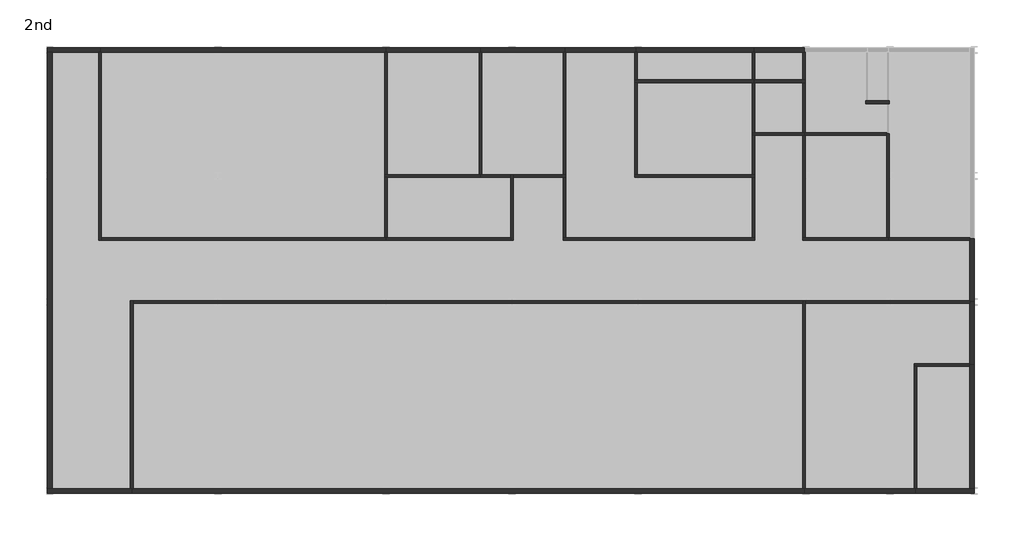
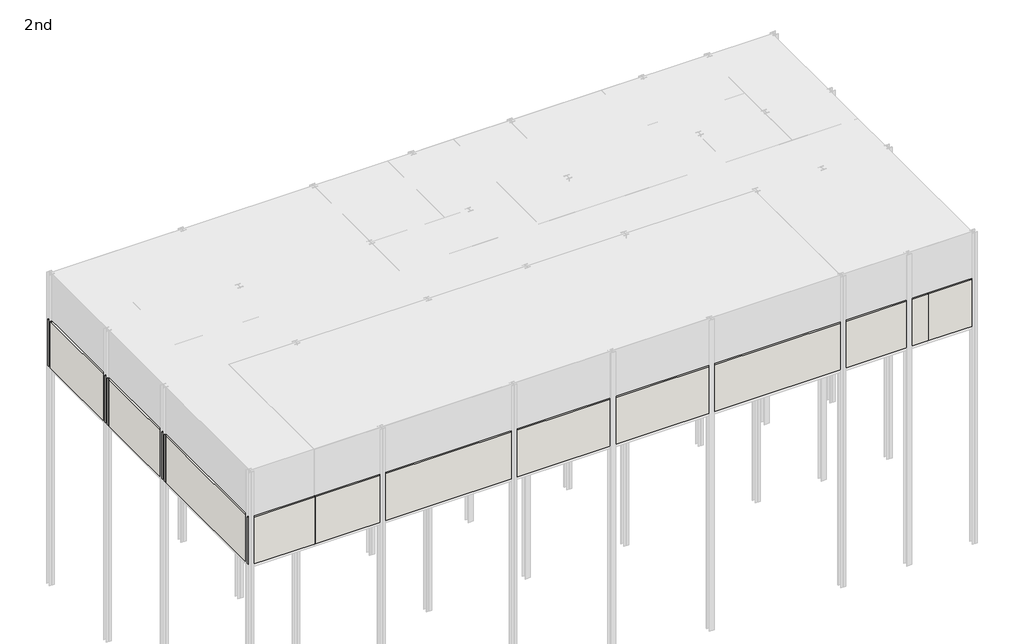
# One storey, part 1 of 3: 52 walls.
"""IFC4 building model written with IfcOpenShell, lengths in millimetres."""

from ifc_helpers import new_model, si_unit, frame, origin, place, context, project, spatial, polyline, outline, extrude, faceted_brep, element, save

model = new_model("IFC4")

# Units and contexts
model_context = context("Model", 3, world=origin())
ifc_project = project(units=[si_unit("LENGTHUNIT", "METRE", prefix="MILLI")], contexts=[model_context])

# Site, building, storey
site = spatial("IfcSite", under=ifc_project)
building = spatial("IfcBuilding", under=site)
storey = spatial("IfcBuildingStorey", under=building, Name="2nd", Elevation=14000.0)

# Walls
placement = place(None, origin())
element("IfcWall", 1, ObjectType="Wall-Ext_215Bwk", at=placement, inside=storey, context=model_context, shape_type="Brep", body=[
    faceted_brep([(160014.1020501, 130908.2581198, 14000.0), (192014.1020501, 130908.2581198, 14000.0), (192014.1020501, 130908.2581198, 17000.0), (160014.1020501, 130908.2581198, 17000.0), (160014.1020501, 131123.2581198, 14000.0), (160014.1020501, 131123.2581198, 17000.0), (160076.6020501, 131123.2581198, 17000.0), (191951.6020501, 131123.2581198, 17000.0), (192014.1020501, 131123.2581198, 17000.0), (192014.1020501, 131123.2581198, 14000.0), (191951.6020501, 131123.2581198, 14000.0), (160076.6020501, 131123.2581198, 14000.0)], [[[0, 1, 2, 3]], [[4, 5, 6, 7, 8, 9, 10, 11]], [[1, 0, 4, 11, 10, 9]], [[2, 1, 9, 8]], [[3, 2, 8, 7, 6, 5]], [[0, 3, 5, 4]]]),
])
element("IfcWall", 2, ObjectType="Wall-Ext_215Bwk", at=placement, inside=storey, context=model_context, shape_type="Brep", body=[
    faceted_brep([(172114.1020501, 152123.2581198, 14000.0), (158514.1020501, 152123.2581198, 14000.0), (158514.1020501, 152123.2581198, 17000.0), (172114.1020501, 152123.2581198, 17000.0), (172114.1020501, 151908.2581198, 14000.0), (172114.1020501, 151908.2581198, 17000.0), (172051.6020501, 151908.2581198, 17000.0), (158576.6020501, 151908.2581198, 17000.0), (158514.1020501, 151908.2581198, 17000.0), (158514.1020501, 151908.2581198, 14000.0), (158576.6020501, 151908.2581198, 14000.0), (172051.6020501, 151908.2581198, 14000.0)], [[[0, 1, 2, 3]], [[4, 5, 6, 7, 8, 9, 10, 11]], [[1, 0, 4, 11, 10, 9]], [[2, 1, 9, 8]], [[3, 2, 8, 7, 6, 5]], [[0, 3, 5, 4]]]),
])
element("IfcWall", 3, ObjectType="Wall-Ext_215Bwk", at=placement, inside=storey, context=model_context, shape_type="Brep", body=[
    faceted_brep([(176614.1020501, 152123.2581198, 14000.0), (172114.1020501, 152123.2581198, 14000.0), (172114.1020501, 152123.2581198, 17000.0), (176614.1020501, 152123.2581198, 17000.0), (176614.1020501, 151908.2581198, 14000.0), (176614.1020501, 151908.2581198, 17000.0), (176551.6020501, 151908.2581198, 17000.0), (172176.6020501, 151908.2581198, 17000.0), (172114.1020501, 151908.2581198, 17000.0), (172114.1020501, 151908.2581198, 14000.0), (172176.6020501, 151908.2581198, 14000.0), (176551.6020501, 151908.2581198, 14000.0)], [[[0, 1, 2, 3]], [[4, 5, 6, 7, 8, 9, 10, 11]], [[1, 0, 4, 11, 10, 9]], [[2, 1, 9, 8]], [[3, 2, 8, 7, 6, 5]], [[0, 3, 5, 4]]]),
])
element("IfcWall", 4, ObjectType="Wall-Ext_215Bwk", at=placement, inside=storey, context=model_context, shape_type="Brep", body=[
    faceted_brep([(180614.1020501, 152123.2581198, 14000.0), (176614.1020501, 152123.2581198, 14000.0), (176614.1020501, 152123.2581198, 17000.0), (180614.1020501, 152123.2581198, 17000.0), (180614.1020501, 151908.2581198, 14000.0), (180614.1020501, 151908.2581198, 17000.0), (180551.6020501, 151908.2581198, 17000.0), (176676.6020501, 151908.2581198, 17000.0), (176614.1020501, 151908.2581198, 17000.0), (176614.1020501, 151908.2581198, 14000.0), (176676.6020501, 151908.2581198, 14000.0), (180551.6020501, 151908.2581198, 14000.0)], [[[0, 1, 2, 3]], [[4, 5, 6, 7, 8, 9, 10, 11]], [[1, 0, 4, 11, 10, 9]], [[2, 1, 9, 8]], [[3, 2, 8, 7, 6, 5]], [[0, 3, 5, 4]]]),
])
element("IfcWall", 5, ObjectType="Wall-Ext_215Bwk", at=placement, inside=storey, context=model_context, shape_type="Brep", body=[
    faceted_brep([(192014.1020501, 152123.2581198, 14000.0), (189614.1020501, 152123.2581198, 14000.0), (189614.1020501, 152123.2581198, 17000.0), (192014.1020501, 152123.2581198, 17000.0), (192014.1020501, 151908.2581198, 14000.0), (192014.1020501, 151908.2581198, 17000.0), (191951.6020501, 151908.2581198, 17000.0), (189676.6020501, 151908.2581198, 17000.0), (189614.1020501, 151908.2581198, 17000.0), (189614.1020501, 151908.2581198, 14000.0), (189676.6020501, 151908.2581198, 14000.0), (191951.6020501, 151908.2581198, 14000.0)], [[[0, 1, 2, 3]], [[4, 5, 6, 7, 8, 9, 10, 11]], [[1, 0, 4, 11, 10, 9]], [[2, 1, 9, 8]], [[3, 2, 8, 7, 6, 5]], [[0, 3, 5, 4]]]),
])
element("IfcWall", 6, ObjectType="Wall-Ext_215Bwk", at=placement, inside=storey, context=model_context, shape_type="Brep", body=[
    faceted_brep([(200121.6020501, 140015.7581198, 14000.0), (200121.6020501, 143015.7581198, 14000.0), (200121.6020501, 143015.7581198, 17000.0), (200121.6020501, 140015.7581198, 17000.0), (199906.6020501, 140015.7581198, 14000.0), (199906.6020501, 140015.7581198, 17000.0), (199906.6020501, 140078.2581198, 17000.0), (199906.6020501, 142953.2581198, 17000.0), (199906.6020501, 143015.7581198, 17000.0), (199906.6020501, 143015.7581198, 14000.0), (199906.6020501, 142953.2581198, 14000.0), (199906.6020501, 140078.2581198, 14000.0)], [[[0, 1, 2, 3]], [[4, 5, 6, 7, 8, 9, 10, 11]], [[1, 0, 4, 11, 10, 9]], [[2, 1, 9, 8]], [[3, 2, 8, 7, 6, 5]], [[0, 3, 5, 4]]]),
])
element("IfcWall", 7, ObjectType="Wall-Ext_215Bwk", at=placement, inside=storey, context=model_context, shape_type="Brep", body=[
    faceted_brep([(158514.1020501, 152123.2581198, 14000.0), (156006.6020501, 152123.2581198, 14000.0), (156006.6020501, 152123.2581198, 17000.0), (158514.1020501, 152123.2581198, 17000.0), (158514.1020501, 151908.2581198, 14000.0), (158514.1020501, 151908.2581198, 17000.0), (158451.6020501, 151908.2581198, 17000.0), (156221.6020501, 151908.2581198, 17000.0), (156006.6020501, 151908.2581198, 17000.0), (156006.6020501, 151908.2581198, 14000.0), (156221.6020501, 151908.2581198, 14000.0), (158451.6020501, 151908.2581198, 14000.0)], [[[0, 1, 2, 3]], [[4, 5, 6, 7, 8, 9, 10, 11]], [[1, 0, 4, 11, 10, 9]], [[3, 2, 8, 7, 6, 5]], [[0, 3, 5, 4]], [[2, 1, 9, 8]]]),
])
element("IfcWall", 8, ObjectType="Wall-Ext_215Bwk", at=placement, inside=storey, context=model_context, shape_type="SweptSolid", body=[
    extrude(outline(polyline([(156006.6020501, 131123.2581198), (156006.6020501, 151908.2581198), (156221.6020501, 151908.2581198), (156221.6020501, 131123.2581198), (156006.6020501, 131123.2581198)])), frame((0.0, 0.0, 14000.0), z_axis=(0.0, 0.0, 1.0), x_axis=(1.0, 0.0, 0.0)), (0.0, 0.0, 1.0), 3000.0),
])
element("IfcWall", 9, ObjectType="Wall-Ext_215Bwk", at=placement, inside=storey, context=model_context, shape_type="Brep", body=[
    faceted_brep([(156006.6020501, 130908.2581198, 14000.0), (160014.1020501, 130908.2581198, 14000.0), (160014.1020501, 130908.2581198, 17000.0), (156006.6020501, 130908.2581198, 17000.0), (156006.6020501, 131123.2581198, 14000.0), (156006.6020501, 131123.2581198, 17000.0), (156221.6020501, 131123.2581198, 17000.0), (159951.6020501, 131123.2581198, 17000.0), (160014.1020501, 131123.2581198, 17000.0), (160014.1020501, 131123.2581198, 14000.0), (159951.6020501, 131123.2581198, 14000.0), (156221.6020501, 131123.2581198, 14000.0)], [[[0, 1, 2, 3]], [[4, 5, 6, 7, 8, 9, 10, 11]], [[1, 0, 4, 11, 10, 9]], [[2, 1, 9, 8]], [[3, 2, 8, 7, 6, 5]], [[0, 3, 5, 4]]]),
])
element("IfcWall", 10, ObjectType="Wall-Ext_215Bwk", at=placement, inside=storey, context=model_context, shape_type="Brep", body=[
    faceted_brep([(189614.1020501, 152123.2581198, 14000.0), (184014.1020501, 152123.2581198, 14000.0), (184014.1020501, 152123.2581198, 17000.0), (189614.1020501, 152123.2581198, 17000.0), (189614.1020501, 151908.2581198, 14000.0), (189614.1020501, 151908.2581198, 17000.0), (189551.6020501, 151908.2581198, 17000.0), (184076.6020501, 151908.2581198, 17000.0), (184014.1020501, 151908.2581198, 17000.0), (184014.1020501, 151908.2581198, 14000.0), (184076.6020501, 151908.2581198, 14000.0), (189551.6020501, 151908.2581198, 14000.0)], [[[0, 1, 2, 3]], [[4, 5, 6, 7, 8, 9, 10, 11]], [[1, 0, 4, 11, 10, 9]], [[2, 1, 9, 8]], [[3, 2, 8, 7, 6, 5]], [[0, 3, 5, 4]]]),
])
element("IfcWall", 11, ObjectType="Wall-Ext_215Bwk", at=placement, inside=storey, context=model_context, shape_type="Brep", body=[
    faceted_brep([(184014.1020501, 152123.2581198, 14000.0), (180614.1020501, 152123.2581198, 14000.0), (180614.1020501, 152123.2581198, 17000.0), (184014.1020501, 152123.2581198, 17000.0), (184014.1020501, 151908.2581198, 14000.0), (184014.1020501, 151908.2581198, 17000.0), (183951.6020501, 151908.2581198, 17000.0), (180676.6020501, 151908.2581198, 17000.0), (180614.1020501, 151908.2581198, 17000.0), (180614.1020501, 151908.2581198, 14000.0), (180676.6020501, 151908.2581198, 14000.0), (183951.6020501, 151908.2581198, 14000.0)], [[[0, 1, 2, 3]], [[4, 5, 6, 7, 8, 9, 10, 11]], [[1, 0, 4, 11, 10, 9]], [[2, 1, 9, 8]], [[3, 2, 8, 7, 6, 5]], [[0, 3, 5, 4]]]),
])
element("IfcWall", 12, ObjectType="Wall-Ext_215Bwk", at=placement, inside=storey, context=model_context, shape_type="Brep", body=[
    faceted_brep([(192014.1020501, 130908.2581198, 14000.0), (197314.1020501, 130908.2581198, 14000.0), (197314.1020501, 130908.2581198, 17000.0), (192014.1020501, 130908.2581198, 17000.0), (192014.1020501, 131123.2581198, 14000.0), (192014.1020501, 131123.2581198, 17000.0), (192076.6020501, 131123.2581198, 17000.0), (197251.6020501, 131123.2581198, 17000.0), (197314.1020501, 131123.2581198, 17000.0), (197314.1020501, 131123.2581198, 14000.0), (197251.6020501, 131123.2581198, 14000.0), (192076.6020501, 131123.2581198, 14000.0)], [[[0, 1, 2, 3]], [[4, 5, 6, 7, 8, 9, 10, 11]], [[1, 0, 4, 11, 10, 9]], [[2, 1, 9, 8]], [[3, 2, 8, 7, 6, 5]], [[0, 3, 5, 4]]]),
])
element("IfcWall", 13, ObjectType="Wall-Ext_215Bwk", at=placement, inside=storey, context=model_context, shape_type="Brep", body=[
    faceted_brep([(200121.6020501, 137015.7581198, 14000.0), (200121.6020501, 140015.7581198, 14000.0), (200121.6020501, 140015.7581198, 17000.0), (200121.6020501, 137015.7581198, 17000.0), (199906.6020501, 137015.7581198, 14000.0), (199906.6020501, 137015.7581198, 17000.0), (199906.6020501, 137078.2581198, 17000.0), (199906.6020501, 139953.2581198, 17000.0), (199906.6020501, 140015.7581198, 17000.0), (199906.6020501, 140015.7581198, 14000.0), (199906.6020501, 139953.2581198, 14000.0), (199906.6020501, 137078.2581198, 14000.0)], [[[0, 1, 2, 3]], [[4, 5, 6, 7, 8, 9, 10, 11]], [[1, 0, 4, 11, 10, 9]], [[2, 1, 9, 8]], [[3, 2, 8, 7, 6, 5]], [[0, 3, 5, 4]]]),
])
element("IfcWall", 14, ObjectType="Wall-Ext_215Bwk", at=placement, inside=storey, context=model_context, shape_type="Brep", body=[
    faceted_brep([(200121.6020501, 131123.2581198, 14000.0), (200121.6020501, 137015.7581198, 14000.0), (200121.6020501, 137015.7581198, 17000.0), (200121.6020501, 131123.2581198, 17000.0), (199906.6020501, 131123.2581198, 14000.0), (199906.6020501, 131123.2581198, 17000.0), (199906.6020501, 136953.2581198, 17000.0), (199906.6020501, 137015.7581198, 17000.0), (199906.6020501, 137015.7581198, 14000.0), (199906.6020501, 136953.2581198, 14000.0)], [[[0, 1, 2, 3]], [[4, 5, 6, 7, 8, 9]], [[1, 0, 4, 9, 8]], [[2, 1, 8, 7]], [[3, 2, 7, 6, 5]], [[0, 3, 5, 4]]]),
])
element("IfcWall", 15, ObjectType="Wall-Ext_215Bwk", at=placement, inside=storey, context=model_context, shape_type="Brep", body=[
    faceted_brep([(197314.1020501, 130908.2581198, 14000.0), (200121.6020501, 130908.2581198, 14000.0), (200121.6020501, 130908.2581198, 17000.0), (197314.1020501, 130908.2581198, 17000.0), (197314.1020501, 131123.2581198, 14000.0), (197314.1020501, 131123.2581198, 17000.0), (197376.6020501, 131123.2581198, 17000.0), (199906.6020501, 131123.2581198, 17000.0), (200121.6020501, 131123.2581198, 17000.0), (200121.6020501, 131123.2581198, 14000.0), (199906.6020501, 131123.2581198, 14000.0), (197376.6020501, 131123.2581198, 14000.0)], [[[0, 1, 2, 3]], [[4, 5, 6, 7, 8, 9, 10, 11]], [[1, 0, 4, 11, 10, 9]], [[3, 2, 8, 7, 6, 5]], [[0, 3, 5, 4]], [[2, 1, 9, 8]]]),
])
element("IfcWall", 16, ObjectType="Wall-Int_12P-100Blk-12P", at=placement, inside=storey, context=model_context, shape_type="SweptSolid", body=[
    extrude(outline(polyline([(160076.6020501, 140078.2581198), (191951.6020501, 140078.2581198), (191951.6020501, 139953.2581198), (160076.6020501, 139953.2581198), (160076.6020501, 140078.2581198)])), frame((0.0, 0.0, 14000.0), z_axis=(0.0, 0.0, 1.0), x_axis=(1.0, 0.0, 0.0)), (0.0, 0.0, 1.0), 3000.0),
])
element("IfcWall", 17, ObjectType="Wall-Int_12P-100Blk-12P", at=placement, inside=storey, context=model_context, shape_type="Brep", body=[
    faceted_brep([(159951.6020501, 140078.2581198, 14000.0), (159951.6020501, 131123.2581198, 14000.0), (159951.6020501, 131123.2581198, 17000.0), (159951.6020501, 140078.2581198, 17000.0), (160076.6020501, 140078.2581198, 14000.0), (160076.6020501, 140078.2581198, 17000.0), (160076.6020501, 139953.2581198, 17000.0), (160076.6020501, 131123.2581198, 17000.0), (160076.6020501, 131123.2581198, 14000.0), (160076.6020501, 139953.2581198, 14000.0), (160014.1020501, 131123.2581198, 14000.0), (160014.1020501, 131123.2581198, 17000.0)], [[[0, 1, 2, 3]], [[4, 5, 6, 7, 8, 9]], [[1, 0, 4, 9, 8, 10]], [[3, 2, 11, 7, 6, 5]], [[0, 3, 5, 4]], [[2, 1, 10, 8, 7, 11]]]),
])
element("IfcWall", 18, ObjectType="Wall-Int_12P-100Blk-12P", at=placement, inside=storey, context=model_context, shape_type="Brep", body=[
    faceted_brep([(192076.6020501, 131123.2581198, 14000.0), (192076.6020501, 139953.2581198, 14000.0), (192076.6020501, 140078.2581198, 14000.0), (192076.6020501, 140078.2581198, 17000.0), (192076.6020501, 139953.2581198, 17000.0), (192076.6020501, 131123.2581198, 17000.0), (191951.6020501, 131123.2581198, 14000.0), (191951.6020501, 131123.2581198, 17000.0), (191951.6020501, 139953.2581198, 17000.0), (191951.6020501, 140078.2581198, 17000.0), (191951.6020501, 140078.2581198, 14000.0), (191951.6020501, 139953.2581198, 14000.0), (192014.1020501, 131123.2581198, 14000.0), (192014.1020501, 131123.2581198, 17000.0)], [[[0, 1, 2, 3, 4, 5]], [[6, 7, 8, 9, 10, 11]], [[2, 1, 0, 12, 6, 11, 10]], [[5, 4, 3, 9, 8, 7, 13]], [[3, 2, 10, 9]], [[0, 5, 13, 7, 6, 12]]]),
])
element("IfcWall", 19, ObjectType="Wall-Int_12P-100Blk-12P", at=placement, inside=storey, context=model_context, shape_type="Brep", body=[
    faceted_brep([(158451.6020501, 151908.2581198, 14000.0), (158451.6020501, 142953.2581198, 14000.0), (158451.6020501, 142953.2581198, 17000.0), (158451.6020501, 151908.2581198, 17000.0), (158576.6020501, 151908.2581198, 14000.0), (158576.6020501, 151908.2581198, 17000.0), (158576.6020501, 143078.2581198, 17000.0), (158576.6020501, 142953.2581198, 17000.0), (158576.6020501, 142953.2581198, 14000.0), (158576.6020501, 143078.2581198, 14000.0), (158514.1020501, 151908.2581198, 14000.0), (158514.1020501, 151908.2581198, 17000.0)], [[[0, 1, 2, 3]], [[4, 5, 6, 7, 8, 9]], [[1, 0, 10, 4, 9, 8]], [[3, 2, 7, 6, 5, 11]], [[0, 3, 11, 5, 4, 10]], [[2, 1, 8, 7]]]),
])
element("IfcWall", 20, ObjectType="Wall-Int_12P-100Blk-12P", at=placement, inside=storey, context=model_context, shape_type="Brep", body=[
    faceted_brep([(158576.6020501, 142953.2581198, 14000.0), (172114.1020501, 142953.2581198, 14000.0), (172114.1020501, 142953.2581198, 17000.0), (158576.6020501, 142953.2581198, 17000.0), (158576.6020501, 143078.2581198, 14000.0), (158576.6020501, 143078.2581198, 17000.0), (172051.6020501, 143078.2581198, 17000.0), (172114.1020501, 143078.2581198, 17000.0), (172114.1020501, 143078.2581198, 14000.0), (172051.6020501, 143078.2581198, 14000.0)], [[[0, 1, 2, 3]], [[4, 5, 6, 7, 8, 9]], [[1, 0, 4, 9, 8]], [[2, 1, 8, 7]], [[3, 2, 7, 6, 5]], [[0, 3, 5, 4]]]),
])
element("IfcWall", 21, ObjectType="Wall-Int_12P-100Blk-12P", at=placement, inside=storey, context=model_context, shape_type="Brep", body=[
    faceted_brep([(172176.6020501, 143078.2581198, 14000.0), (172176.6020501, 145953.2581198, 14000.0), (172176.6020501, 145953.2581198, 17000.0), (172176.6020501, 143078.2581198, 17000.0), (172051.6020501, 143078.2581198, 14000.0), (172051.6020501, 143078.2581198, 17000.0), (172051.6020501, 145953.2581198, 17000.0), (172051.6020501, 145953.2581198, 14000.0), (172114.1020501, 143078.2581198, 14000.0), (172114.1020501, 143078.2581198, 17000.0)], [[[0, 1, 2, 3]], [[4, 5, 6, 7]], [[1, 0, 8, 4, 7]], [[3, 2, 6, 5, 9]], [[0, 3, 9, 5, 4, 8]], [[2, 1, 7, 6]]]),
])
element("IfcWall", 22, ObjectType="Wall-Int_12P-100Blk-12P", at=placement, inside=storey, context=model_context, shape_type="Brep", body=[
    faceted_brep([(172176.6020501, 146078.2581198, 14000.0), (172176.6020501, 151908.2581198, 14000.0), (172176.6020501, 151908.2581198, 17000.0), (172176.6020501, 146078.2581198, 17000.0), (172051.6020501, 146078.2581198, 14000.0), (172051.6020501, 146078.2581198, 17000.0), (172051.6020501, 151908.2581198, 17000.0), (172051.6020501, 151908.2581198, 14000.0), (172114.1020501, 151908.2581198, 14000.0), (172114.1020501, 151908.2581198, 17000.0)], [[[0, 1, 2, 3]], [[4, 5, 6, 7]], [[1, 0, 4, 7, 8]], [[3, 2, 9, 6, 5]], [[2, 1, 8, 7, 6, 9]], [[0, 3, 5, 4]]]),
])
element("IfcWall", 23, ObjectType="Wall-Int_12P-100Blk-12P", at=placement, inside=storey, context=model_context, shape_type="Brep", body=[
    faceted_brep([(172051.6020501, 145953.2581198, 14000.0), (172176.6020501, 145953.2581198, 14000.0), (176614.1020501, 145953.2581198, 14000.0), (176614.1020501, 145953.2581198, 17000.0), (172176.6020501, 145953.2581198, 17000.0), (172051.6020501, 145953.2581198, 17000.0), (172051.6020501, 146078.2581198, 14000.0), (172051.6020501, 146078.2581198, 17000.0), (172176.6020501, 146078.2581198, 17000.0), (176551.6020501, 146078.2581198, 17000.0), (176614.1020501, 146078.2581198, 17000.0), (176614.1020501, 146078.2581198, 14000.0), (176551.6020501, 146078.2581198, 14000.0), (172176.6020501, 146078.2581198, 14000.0)], [[[0, 1, 2, 3, 4, 5]], [[6, 7, 8, 9, 10, 11, 12, 13]], [[2, 1, 0, 6, 13, 12, 11]], [[3, 2, 11, 10]], [[5, 4, 3, 10, 9, 8, 7]], [[0, 5, 7, 6]]]),
])
element("IfcWall", 24, ObjectType="Wall-Int_12P-100Blk-12P", at=placement, inside=storey, context=model_context, shape_type="Brep", body=[
    faceted_brep([(176676.6020501, 146078.2581198, 14000.0), (176676.6020501, 151908.2581198, 14000.0), (176676.6020501, 151908.2581198, 17000.0), (176676.6020501, 146078.2581198, 17000.0), (176551.6020501, 146078.2581198, 14000.0), (176551.6020501, 146078.2581198, 17000.0), (176551.6020501, 151908.2581198, 17000.0), (176551.6020501, 151908.2581198, 14000.0), (176614.1020501, 146078.2581198, 14000.0), (176614.1020501, 151908.2581198, 14000.0), (176614.1020501, 151908.2581198, 17000.0), (176614.1020501, 146078.2581198, 17000.0)], [[[0, 1, 2, 3]], [[4, 5, 6, 7]], [[1, 0, 8, 4, 7, 9]], [[3, 2, 10, 6, 5, 11]], [[2, 1, 9, 7, 6, 10]], [[0, 3, 11, 5, 4, 8]]]),
])
element("IfcWall", 25, ObjectType="Wall-Int_12P-100Blk-12P", at=placement, inside=storey, context=model_context, shape_type="Brep", body=[
    faceted_brep([(191951.6020501, 147953.2581198, 14000.0), (191951.6020501, 143078.2581198, 14000.0), (191951.6020501, 143078.2581198, 17000.0), (191951.6020501, 147953.2581198, 17000.0), (192076.6020501, 147953.2581198, 14000.0), (192076.6020501, 147953.2581198, 17000.0), (192076.6020501, 143078.2581198, 17000.0), (192076.6020501, 143078.2581198, 14000.0), (192014.1020501, 147953.2581198, 14000.0), (192014.1020501, 147953.2581198, 17000.0)], [[[0, 1, 2, 3]], [[4, 5, 6, 7]], [[1, 0, 8, 4, 7]], [[3, 2, 6, 5, 9]], [[0, 3, 9, 5, 4, 8]], [[2, 1, 7, 6]]]),
])
element("IfcWall", 26, ObjectType="Wall-Int_12P-100Blk-12P", at=placement, inside=storey, context=model_context, shape_type="Brep", body=[
    faceted_brep([(191951.6020501, 142953.2581198, 14000.0), (196014.1020501, 142953.2581198, 14000.0), (196014.1020501, 142953.2581198, 17000.0), (191951.6020501, 142953.2581198, 17000.0), (191951.6020501, 143078.2581198, 14000.0), (191951.6020501, 143078.2581198, 17000.0), (192076.6020501, 143078.2581198, 17000.0), (195951.6020501, 143078.2581198, 17000.0), (196014.1020501, 143078.2581198, 17000.0), (196014.1020501, 143078.2581198, 14000.0), (195951.6020501, 143078.2581198, 14000.0), (192076.6020501, 143078.2581198, 14000.0)], [[[0, 1, 2, 3]], [[4, 5, 6, 7, 8, 9, 10, 11]], [[1, 0, 4, 11, 10, 9]], [[2, 1, 9, 8]], [[3, 2, 8, 7, 6, 5]], [[0, 3, 5, 4]]]),
])
element("IfcWall", 27, ObjectType="Wall-Int_12P-100Blk-12P", at=placement, inside=storey, context=model_context, shape_type="Brep", body=[
    faceted_brep([(196076.6020501, 143078.2581198, 14000.0), (196076.6020501, 148015.7581198, 14000.0), (196076.6020501, 148015.7581198, 17000.0), (196076.6020501, 143078.2581198, 17000.0), (195951.6020501, 143078.2581198, 14000.0), (195951.6020501, 143078.2581198, 17000.0), (195951.6020501, 147953.2581198, 17000.0), (195951.6020501, 148015.7581198, 17000.0), (195951.6020501, 148015.7581198, 14000.0), (195951.6020501, 147953.2581198, 14000.0), (196014.1020501, 143078.2581198, 14000.0), (196014.1020501, 143078.2581198, 17000.0)], [[[0, 1, 2, 3]], [[4, 5, 6, 7, 8, 9]], [[1, 0, 10, 4, 9, 8]], [[2, 1, 8, 7]], [[3, 2, 7, 6, 5, 11]], [[0, 3, 11, 5, 4, 10]]]),
])
element("IfcWall", 28, ObjectType="Wall-Int_12P-100Blk-12P", at=placement, inside=storey, context=model_context, shape_type="Brep", body=[
    faceted_brep([(195951.6020501, 148078.2581198, 14000.0), (192076.6020501, 148078.2581198, 14000.0), (192014.1020501, 148078.2581198, 14000.0), (192014.1020501, 148078.2581198, 17000.0), (192076.6020501, 148078.2581198, 17000.0), (195951.6020501, 148078.2581198, 17000.0), (195951.6020501, 147953.2581198, 14000.0), (195951.6020501, 147953.2581198, 17000.0), (192076.6020501, 147953.2581198, 17000.0), (192014.1020501, 147953.2581198, 17000.0), (192014.1020501, 147953.2581198, 14000.0), (192076.6020501, 147953.2581198, 14000.0), (195951.6020501, 148015.7581198, 14000.0), (195951.6020501, 148015.7581198, 17000.0)], [[[0, 1, 2, 3, 4, 5]], [[6, 7, 8, 9, 10, 11]], [[2, 1, 0, 12, 6, 11, 10]], [[3, 2, 10, 9]], [[5, 4, 3, 9, 8, 7, 13]], [[0, 5, 13, 7, 6, 12]]]),
])
element("IfcWall", 29, ObjectType="Wall-Int_12P-100Blk-12P", at=placement, inside=storey, context=model_context, shape_type="Brep", body=[
    faceted_brep([(196014.1020501, 142953.2581198, 14000.0), (199906.6020501, 142953.2581198, 14000.0), (199906.6020501, 142953.2581198, 17000.0), (196014.1020501, 142953.2581198, 17000.0), (196014.1020501, 143078.2581198, 14000.0), (196014.1020501, 143078.2581198, 17000.0), (196076.6020501, 143078.2581198, 17000.0), (199906.6020501, 143078.2581198, 17000.0), (199906.6020501, 143078.2581198, 14000.0), (196076.6020501, 143078.2581198, 14000.0), (199906.6020501, 143015.7581198, 14000.0), (199906.6020501, 143015.7581198, 17000.0)], [[[0, 1, 2, 3]], [[4, 5, 6, 7, 8, 9]], [[1, 0, 4, 9, 8, 10]], [[3, 2, 11, 7, 6, 5]], [[0, 3, 5, 4]], [[2, 1, 10, 8, 7, 11]]]),
])
element("IfcWall", 30, ObjectType="Wall-Int_12P-100Blk-12P", at=placement, inside=storey, context=model_context, shape_type="Brep", body=[
    faceted_brep([(176614.1020501, 145953.2581198, 14000.0), (178051.6020501, 145953.2581198, 14000.0), (178051.6020501, 145953.2581198, 17000.0), (176614.1020501, 145953.2581198, 17000.0), (176614.1020501, 146078.2581198, 14000.0), (176614.1020501, 146078.2581198, 17000.0), (176676.6020501, 146078.2581198, 17000.0), (178051.6020501, 146078.2581198, 17000.0), (178051.6020501, 146078.2581198, 14000.0), (176676.6020501, 146078.2581198, 14000.0)], [[[0, 1, 2, 3]], [[4, 5, 6, 7, 8, 9]], [[1, 0, 4, 9, 8]], [[3, 2, 7, 6, 5]], [[0, 3, 5, 4]], [[2, 1, 8, 7]]]),
])
element("IfcWall", 31, ObjectType="Wall-Int_12P-100Blk-12P", at=placement, inside=storey, context=model_context, shape_type="Brep", body=[
    faceted_brep([(178176.6020501, 145953.2581198, 14000.0), (180551.6020501, 145953.2581198, 14000.0), (180676.6020501, 145953.2581198, 14000.0), (180676.6020501, 145953.2581198, 17000.0), (180551.6020501, 145953.2581198, 17000.0), (178176.6020501, 145953.2581198, 17000.0), (178176.6020501, 146078.2581198, 14000.0), (178176.6020501, 146078.2581198, 17000.0), (180551.6020501, 146078.2581198, 17000.0), (180676.6020501, 146078.2581198, 17000.0), (180676.6020501, 146078.2581198, 14000.0), (180551.6020501, 146078.2581198, 14000.0)], [[[0, 1, 2, 3, 4, 5]], [[6, 7, 8, 9, 10, 11]], [[2, 1, 0, 6, 11, 10]], [[5, 4, 3, 9, 8, 7]], [[3, 2, 10, 9]], [[0, 5, 7, 6]]]),
])
element("IfcWall", 32, ObjectType="Wall-Int_12P-100Blk-12P", at=placement, inside=storey, context=model_context, shape_type="Brep", body=[
    faceted_brep([(180676.6020501, 146078.2581198, 14000.0), (180676.6020501, 151908.2581198, 14000.0), (180676.6020501, 151908.2581198, 17000.0), (180676.6020501, 146078.2581198, 17000.0), (180551.6020501, 146078.2581198, 14000.0), (180551.6020501, 146078.2581198, 17000.0), (180551.6020501, 151908.2581198, 17000.0), (180551.6020501, 151908.2581198, 14000.0), (180614.1020501, 151908.2581198, 14000.0), (180614.1020501, 151908.2581198, 17000.0)], [[[0, 1, 2, 3]], [[4, 5, 6, 7]], [[1, 0, 4, 7, 8]], [[3, 2, 9, 6, 5]], [[2, 1, 8, 7, 6, 9]], [[0, 3, 5, 4]]]),
])
element("IfcWall", 33, ObjectType="Wall-Int_12P-100Blk-12P", at=placement, inside=storey, context=model_context, shape_type="Brep", body=[
    faceted_brep([(172114.1020501, 142953.2581198, 14000.0), (178051.6020501, 142953.2581198, 14000.0), (178051.6020501, 142953.2581198, 17000.0), (172114.1020501, 142953.2581198, 17000.0), (172114.1020501, 143078.2581198, 14000.0), (172114.1020501, 143078.2581198, 17000.0), (172176.6020501, 143078.2581198, 17000.0), (178051.6020501, 143078.2581198, 17000.0), (178051.6020501, 143078.2581198, 14000.0), (172176.6020501, 143078.2581198, 14000.0)], [[[0, 1, 2, 3]], [[4, 5, 6, 7, 8, 9]], [[1, 0, 4, 9, 8]], [[3, 2, 7, 6, 5]], [[0, 3, 5, 4]], [[2, 1, 8, 7]]]),
])
element("IfcWall", 34, ObjectType="Wall-Int_12P-100Blk-12P", at=placement, inside=storey, context=model_context, shape_type="Brep", body=[
    faceted_brep([(178176.6020501, 142953.2581198, 14000.0), (178176.6020501, 145953.2581198, 14000.0), (178176.6020501, 146078.2581198, 14000.0), (178176.6020501, 146078.2581198, 17000.0), (178176.6020501, 145953.2581198, 17000.0), (178176.6020501, 142953.2581198, 17000.0), (178051.6020501, 142953.2581198, 14000.0), (178051.6020501, 142953.2581198, 17000.0), (178051.6020501, 143078.2581198, 17000.0), (178051.6020501, 145953.2581198, 17000.0), (178051.6020501, 146078.2581198, 17000.0), (178051.6020501, 146078.2581198, 14000.0), (178051.6020501, 145953.2581198, 14000.0), (178051.6020501, 143078.2581198, 14000.0)], [[[0, 1, 2, 3, 4, 5]], [[6, 7, 8, 9, 10, 11, 12, 13]], [[2, 1, 0, 6, 13, 12, 11]], [[5, 4, 3, 10, 9, 8, 7]], [[0, 5, 7, 6]], [[3, 2, 11, 10]]]),
])
element("IfcWall", 35, ObjectType="Wall-Int_12P-100Blk-12P", at=placement, inside=storey, context=model_context, shape_type="Brep", body=[
    faceted_brep([(189551.6020501, 151908.2581198, 14000.0), (189551.6020501, 150578.2581198, 14000.0), (189551.6020501, 150578.2581198, 17000.0), (189551.6020501, 151908.2581198, 17000.0), (189676.6020501, 151908.2581198, 14000.0), (189676.6020501, 151908.2581198, 17000.0), (189676.6020501, 150578.2581198, 17000.0), (189676.6020501, 150578.2581198, 14000.0), (189614.1020501, 151908.2581198, 14000.0), (189614.1020501, 150578.2581198, 14000.0), (189614.1020501, 150578.2581198, 17000.0), (189614.1020501, 151908.2581198, 17000.0)], [[[0, 1, 2, 3]], [[4, 5, 6, 7]], [[1, 0, 8, 4, 7, 9]], [[3, 2, 10, 6, 5, 11]], [[0, 3, 11, 5, 4, 8]], [[2, 1, 9, 7, 6, 10]]]),
])
element("IfcWall", 36, ObjectType="Wall-Int_12P-100Blk-12P", at=placement, inside=storey, context=model_context, shape_type="Brep", body=[
    faceted_brep([(189614.1020501, 150453.2581198, 14000.0), (189676.6020501, 150453.2581198, 14000.0), (191951.6020501, 150453.2581198, 14000.0), (192076.6020501, 150453.2581198, 14000.0), (192076.6020501, 150453.2581198, 17000.0), (191951.6020501, 150453.2581198, 17000.0), (189676.6020501, 150453.2581198, 17000.0), (189614.1020501, 150453.2581198, 17000.0), (189614.1020501, 150578.2581198, 14000.0), (189614.1020501, 150578.2581198, 17000.0), (189676.6020501, 150578.2581198, 17000.0), (191951.6020501, 150578.2581198, 17000.0), (192076.6020501, 150578.2581198, 17000.0), (192076.6020501, 150578.2581198, 14000.0), (191951.6020501, 150578.2581198, 14000.0), (189676.6020501, 150578.2581198, 14000.0)], [[[0, 1, 2, 3, 4, 5, 6, 7]], [[8, 9, 10, 11, 12, 13, 14, 15]], [[3, 2, 1, 0, 8, 15, 14, 13]], [[7, 6, 5, 4, 12, 11, 10, 9]], [[0, 7, 9, 8]], [[4, 3, 13, 12]]]),
])
element("IfcWall", 37, ObjectType="Wall-Int_12P-100Blk-12P", at=placement, inside=storey, context=model_context, shape_type="Brep", body=[
    faceted_brep([(192076.6020501, 150578.2581198, 14000.0), (192076.6020501, 151908.2581198, 14000.0), (192076.6020501, 151908.2581198, 17000.0), (192076.6020501, 150578.2581198, 17000.0), (191951.6020501, 150578.2581198, 14000.0), (191951.6020501, 150578.2581198, 17000.0), (191951.6020501, 151908.2581198, 17000.0), (191951.6020501, 151908.2581198, 14000.0), (192014.1020501, 151908.2581198, 14000.0), (192014.1020501, 151908.2581198, 17000.0)], [[[0, 1, 2, 3]], [[4, 5, 6, 7]], [[1, 0, 4, 7, 8]], [[3, 2, 9, 6, 5]], [[2, 1, 8, 7, 6, 9]], [[0, 3, 5, 4]]]),
])
element("IfcWall", 38, ObjectType="Wall-Int_12P-100Blk-12P", at=placement, inside=storey, context=model_context, shape_type="Brep", body=[
    faceted_brep([(192076.6020501, 139953.2581198, 14000.0), (199906.6020501, 139953.2581198, 14000.0), (199906.6020501, 139953.2581198, 17000.0), (192076.6020501, 139953.2581198, 17000.0), (192076.6020501, 140078.2581198, 14000.0), (192076.6020501, 140078.2581198, 17000.0), (199906.6020501, 140078.2581198, 17000.0), (199906.6020501, 140078.2581198, 14000.0), (199906.6020501, 140015.7581198, 14000.0), (199906.6020501, 140015.7581198, 17000.0)], [[[0, 1, 2, 3]], [[4, 5, 6, 7]], [[1, 0, 4, 7, 8]], [[3, 2, 9, 6, 5]], [[0, 3, 5, 4]], [[2, 1, 8, 7, 6, 9]]]),
])
element("IfcWall", 39, ObjectType="Wall-Int_12P-100Blk-12P", at=placement, inside=storey, context=model_context, shape_type="Brep", body=[
    faceted_brep([(192014.1020501, 148078.2581198, 14000.0), (191951.6020501, 148078.2581198, 14000.0), (189676.6020501, 148078.2581198, 14000.0), (189551.6020501, 148078.2581198, 14000.0), (189551.6020501, 148078.2581198, 17000.0), (189676.6020501, 148078.2581198, 17000.0), (191951.6020501, 148078.2581198, 17000.0), (192014.1020501, 148078.2581198, 17000.0), (192014.1020501, 147953.2581198, 14000.0), (192014.1020501, 147953.2581198, 17000.0), (191951.6020501, 147953.2581198, 17000.0), (189676.6020501, 147953.2581198, 17000.0), (189551.6020501, 147953.2581198, 17000.0), (189551.6020501, 147953.2581198, 14000.0), (189676.6020501, 147953.2581198, 14000.0), (191951.6020501, 147953.2581198, 14000.0)], [[[0, 1, 2, 3, 4, 5, 6, 7]], [[8, 9, 10, 11, 12, 13, 14, 15]], [[3, 2, 1, 0, 8, 15, 14, 13]], [[7, 6, 5, 4, 12, 11, 10, 9]], [[0, 7, 9, 8]], [[4, 3, 13, 12]]]),
])
element("IfcWall", 40, ObjectType="Wall-Int_12P-100Blk-12P", at=placement, inside=storey, context=model_context, shape_type="SweptSolid", body=[
    extrude(outline(polyline([(189551.6020501, 146078.2581198), (189551.6020501, 147953.2581198), (189676.6020501, 147953.2581198), (189676.6020501, 146078.2581198), (189551.6020501, 146078.2581198)])), frame((0.0, 0.0, 14000.0), z_axis=(0.0, 0.0, 1.0), x_axis=(1.0, 0.0, 0.0)), (0.0, 0.0, 1.0), 3000.0),
])
element("IfcWall", 41, ObjectType="Wall-Int_12P-100Blk-12P", at=placement, inside=storey, context=model_context, shape_type="SweptSolid", body=[
    extrude(outline(polyline([(189551.6020501, 143078.2581198), (189551.6020501, 145953.2581198), (189676.6020501, 145953.2581198), (189676.6020501, 143078.2581198), (189551.6020501, 143078.2581198)])), frame((0.0, 0.0, 14000.0), z_axis=(0.0, 0.0, 1.0), x_axis=(1.0, 0.0, 0.0)), (0.0, 0.0, 1.0), 3000.0),
])
element("IfcWall", 42, ObjectType="Wall-Int_12P-100Blk-12P", at=placement, inside=storey, context=model_context, shape_type="Brep", body=[
    faceted_brep([(189676.6020501, 143078.2581198, 14000.0), (189551.6020501, 143078.2581198, 14000.0), (180676.6020501, 143078.2581198, 14000.0), (180551.6020501, 143078.2581198, 14000.0), (180551.6020501, 143078.2581198, 17000.0), (180676.6020501, 143078.2581198, 17000.0), (189551.6020501, 143078.2581198, 17000.0), (189676.6020501, 143078.2581198, 17000.0), (189676.6020501, 142953.2581198, 14000.0), (189676.6020501, 142953.2581198, 17000.0), (180551.6020501, 142953.2581198, 17000.0), (180551.6020501, 142953.2581198, 14000.0)], [[[0, 1, 2, 3, 4, 5, 6, 7]], [[8, 9, 10, 11]], [[3, 2, 1, 0, 8, 11]], [[7, 6, 5, 4, 10, 9]], [[0, 7, 9, 8]], [[4, 3, 11, 10]]]),
])
element("IfcWall", 43, ObjectType="Wall-Int_12P-100Blk-12P", at=placement, inside=storey, context=model_context, shape_type="SweptSolid", body=[
    extrude(outline(polyline([(180676.6020501, 145953.2581198), (180676.6020501, 143078.2581198), (180551.6020501, 143078.2581198), (180551.6020501, 145953.2581198), (180676.6020501, 145953.2581198)])), frame((0.0, 0.0, 14000.0), z_axis=(0.0, 0.0, 1.0), x_axis=(1.0, 0.0, 0.0)), (0.0, 0.0, 1.0), 3000.0),
])
element("IfcWall", 44, ObjectType="Wall-Int_12P-100Blk-12P", at=placement, inside=storey, context=model_context, shape_type="Brep", body=[
    faceted_brep([(189551.6020501, 150453.2581198, 14000.0), (189551.6020501, 148078.2581198, 14000.0), (189551.6020501, 148078.2581198, 17000.0), (189551.6020501, 150453.2581198, 17000.0), (189676.6020501, 150453.2581198, 14000.0), (189676.6020501, 150453.2581198, 17000.0), (189676.6020501, 148078.2581198, 17000.0), (189676.6020501, 148078.2581198, 14000.0), (189614.1020501, 150453.2581198, 14000.0), (189614.1020501, 150453.2581198, 17000.0)], [[[0, 1, 2, 3]], [[4, 5, 6, 7]], [[1, 0, 8, 4, 7]], [[3, 2, 6, 5, 9]], [[0, 3, 9, 5, 4, 8]], [[2, 1, 7, 6]]]),
])
element("IfcWall", 45, ObjectType="Wall-Int_12P-100Blk-12P", at=placement, inside=storey, context=model_context, shape_type="Brep", body=[
    faceted_brep([(192076.6020501, 148078.2581198, 14000.0), (192076.6020501, 150453.2581198, 14000.0), (192076.6020501, 150453.2581198, 17000.0), (192076.6020501, 148078.2581198, 17000.0), (191951.6020501, 148078.2581198, 14000.0), (191951.6020501, 148078.2581198, 17000.0), (191951.6020501, 150453.2581198, 17000.0), (191951.6020501, 150453.2581198, 14000.0), (192014.1020501, 148078.2581198, 14000.0), (192014.1020501, 148078.2581198, 17000.0)], [[[0, 1, 2, 3]], [[4, 5, 6, 7]], [[1, 0, 8, 4, 7]], [[3, 2, 6, 5, 9]], [[0, 3, 9, 5, 4, 8]], [[2, 1, 7, 6]]]),
])
element("IfcWall", 46, ObjectType="Wall-Int_12P-100Blk-12P", at=placement, inside=storey, context=model_context, shape_type="Brep", body=[
    faceted_brep([(183951.6020501, 151908.2581198, 14000.0), (183951.6020501, 150578.2581198, 14000.0), (183951.6020501, 150578.2581198, 17000.0), (183951.6020501, 151908.2581198, 17000.0), (184076.6020501, 151908.2581198, 14000.0), (184076.6020501, 151908.2581198, 17000.0), (184076.6020501, 150578.2581198, 17000.0), (184076.6020501, 150578.2581198, 14000.0), (184014.1020501, 151908.2581198, 14000.0), (184014.1020501, 151908.2581198, 17000.0)], [[[0, 1, 2, 3]], [[4, 5, 6, 7]], [[1, 0, 8, 4, 7]], [[3, 2, 6, 5, 9]], [[0, 3, 9, 5, 4, 8]], [[2, 1, 7, 6]]]),
])
element("IfcWall", 47, ObjectType="Wall-Int_12P-100Blk-12P", at=placement, inside=storey, context=model_context, shape_type="Brep", body=[
    faceted_brep([(183951.6020501, 150453.2581198, 14000.0), (184076.6020501, 150453.2581198, 14000.0), (189551.6020501, 150453.2581198, 14000.0), (189614.1020501, 150453.2581198, 14000.0), (189614.1020501, 150453.2581198, 17000.0), (189551.6020501, 150453.2581198, 17000.0), (184076.6020501, 150453.2581198, 17000.0), (183951.6020501, 150453.2581198, 17000.0), (183951.6020501, 150578.2581198, 14000.0), (183951.6020501, 150578.2581198, 17000.0), (184076.6020501, 150578.2581198, 17000.0), (189551.6020501, 150578.2581198, 17000.0), (189614.1020501, 150578.2581198, 17000.0), (189614.1020501, 150578.2581198, 14000.0), (189551.6020501, 150578.2581198, 14000.0), (184076.6020501, 150578.2581198, 14000.0)], [[[0, 1, 2, 3, 4, 5, 6, 7]], [[8, 9, 10, 11, 12, 13, 14, 15]], [[3, 2, 1, 0, 8, 15, 14, 13]], [[4, 3, 13, 12]], [[7, 6, 5, 4, 12, 11, 10, 9]], [[0, 7, 9, 8]]]),
])
element("IfcWall", 48, ObjectType="Wall-Int_12P-100Blk-12P", at=placement, inside=storey, context=model_context, shape_type="Brep", body=[
    faceted_brep([(189676.6020501, 146078.2581198, 14000.0), (189551.6020501, 146078.2581198, 14000.0), (184076.6020501, 146078.2581198, 14000.0), (183951.6020501, 146078.2581198, 14000.0), (183951.6020501, 146078.2581198, 17000.0), (184076.6020501, 146078.2581198, 17000.0), (189551.6020501, 146078.2581198, 17000.0), (189676.6020501, 146078.2581198, 17000.0), (189676.6020501, 145953.2581198, 14000.0), (189676.6020501, 145953.2581198, 17000.0), (189551.6020501, 145953.2581198, 17000.0), (183951.6020501, 145953.2581198, 17000.0), (183951.6020501, 145953.2581198, 14000.0), (189551.6020501, 145953.2581198, 14000.0)], [[[0, 1, 2, 3, 4, 5, 6, 7]], [[8, 9, 10, 11, 12, 13]], [[3, 2, 1, 0, 8, 13, 12]], [[7, 6, 5, 4, 11, 10, 9]], [[4, 3, 12, 11]], [[0, 7, 9, 8]]]),
])
element("IfcWall", 49, ObjectType="Wall-Int_12P-100Blk-12P", at=placement, inside=storey, context=model_context, shape_type="SweptSolid", body=[
    extrude(outline(polyline([(184076.6020501, 150453.2581198), (184076.6020501, 146078.2581198), (183951.6020501, 146078.2581198), (183951.6020501, 150453.2581198), (184076.6020501, 150453.2581198)])), frame((0.0, 0.0, 14000.0), z_axis=(0.0, 0.0, 1.0), x_axis=(1.0, 0.0, 0.0)), (0.0, 0.0, 1.0), 3000.0),
])
element("IfcWall", 50, ObjectType="Wall-Int_12P-100Blk-12P", at=placement, inside=storey, context=model_context, shape_type="Brep", body=[
    faceted_brep([(197376.6020501, 131123.2581198, 14000.0), (197376.6020501, 136953.2581198, 14000.0), (197376.6020501, 136953.2581198, 17000.0), (197376.6020501, 131123.2581198, 17000.0), (197251.6020501, 131123.2581198, 14000.0), (197251.6020501, 131123.2581198, 17000.0), (197251.6020501, 136953.2581198, 17000.0), (197251.6020501, 136953.2581198, 14000.0), (197314.1020501, 131123.2581198, 14000.0), (197314.1020501, 131123.2581198, 17000.0)], [[[0, 1, 2, 3]], [[4, 5, 6, 7]], [[1, 0, 8, 4, 7]], [[3, 2, 6, 5, 9]], [[2, 1, 7, 6]], [[0, 3, 9, 5, 4, 8]]]),
])
element("IfcWall", 51, ObjectType="Wall-Int_12P-100Blk-12P", at=placement, inside=storey, context=model_context, shape_type="Brep", body=[
    faceted_brep([(197251.6020501, 136953.2581198, 14000.0), (197376.6020501, 136953.2581198, 14000.0), (199906.6020501, 136953.2581198, 14000.0), (199906.6020501, 136953.2581198, 17000.0), (197376.6020501, 136953.2581198, 17000.0), (197251.6020501, 136953.2581198, 17000.0), (197251.6020501, 137078.2581198, 14000.0), (197251.6020501, 137078.2581198, 17000.0), (199906.6020501, 137078.2581198, 17000.0), (199906.6020501, 137078.2581198, 14000.0), (199906.6020501, 137015.7581198, 14000.0), (199906.6020501, 137015.7581198, 17000.0)], [[[0, 1, 2, 3, 4, 5]], [[6, 7, 8, 9]], [[2, 1, 0, 6, 9, 10]], [[5, 4, 3, 11, 8, 7]], [[0, 5, 7, 6]], [[3, 2, 10, 9, 8, 11]]]),
])
element("IfcWall", 52, ObjectType="Wall-Int_12P-100Blk-12P", at=placement, inside=storey, context=model_context, shape_type="Brep", body=[
    faceted_brep([(196076.6020501, 149578.2581198, 14000.0), (195951.6020501, 149578.2581198, 14000.0), (195076.6020501, 149578.2581198, 14000.0), (194951.6020501, 149578.2581198, 14000.0), (194951.6020501, 149578.2581198, 17000.0), (195076.6020501, 149578.2581198, 17000.0), (195951.6020501, 149578.2581198, 17000.0), (196076.6020501, 149578.2581198, 17000.0), (196076.6020501, 149453.2581198, 14000.0), (196076.6020501, 149453.2581198, 17000.0), (195951.6020501, 149453.2581198, 17000.0), (194951.6020501, 149453.2581198, 17000.0), (194951.6020501, 149453.2581198, 14000.0), (195951.6020501, 149453.2581198, 14000.0)], [[[0, 1, 2, 3, 4, 5, 6, 7]], [[8, 9, 10, 11, 12, 13]], [[3, 2, 1, 0, 8, 13, 12]], [[7, 6, 5, 4, 11, 10, 9]], [[4, 3, 12, 11]], [[0, 7, 9, 8]]]),
])

save(model, "model.ifc")

# Revit data of these elements
# Type "Wall-Ext_215Bwk"
#   Keynote = "F10"
#   Layers, outside or top first: 215 mm "Brick, Common" (function 1)
# Type "Wall-Int_12P-100Blk-12P"
#   Layers, outside or top first: 12.5 mm "Plaster" (function 5); 100 mm "Concrete Masonry Units" (function 1); 12.5 mm "Plaster" (function 5)
# Elements 1, 2, 3, 4, 5, 6, 7, 8, 9, 10, 11, 12, 13, 14, 15 (IfcWall, "Wall-Ext_215Bwk")
#   Top Offset = 0 mm
#   Base Offset = 0 mm
#   Unconnected Height = 3000 mm
#   wall height = 3000 mm
#   Phase Created = New Construction
#   Base Constraint = 2nd
#   Materials on its faces: "Brick, Common"
# Elements 16, 20, 21, 22, 24, 25, 27, 28, 29, 30, 32, 33, 35, 37, 38, 40, 41, 43, 44, 45, 46, 49, 50 (IfcWall, "Wall-Int_12P-100Blk-12P")
#   Top Offset = 0 mm
#   Base Offset = 0 mm
#   Unconnected Height = 3000 mm
#   wall height = 3000 mm
#   Phase Created = New Construction
#   Base Constraint = 2nd
#   Materials on its faces: "Default Wall", "Plaster"
# Elements 17, 18, 19, 23, 26, 31, 34, 36, 39, 42, 47, 48, 51, 52 (IfcWall, "Wall-Int_12P-100Blk-12P")
#   Top Offset = 0 mm
#   Base Offset = 0 mm
#   Unconnected Height = 3000 mm
#   wall height = 3000 mm
#   Phase Created = New Construction
#   Base Constraint = 2nd
#   Materials on its faces: "Plaster", "Default Wall"
# Materials
#   "Brick, Common": class "Masonry", colour RGB 170 100 105, transparency 0, Description = "Common brick", Cost = 0
#   "Plaster": class "Generic", colour RGB 249 249 249, transparency 0, Description = "Plaster", Cost = 0
#   "Concrete Masonry Units": class "Masonry", colour RGB 181 181 181, transparency 0, Description = "Concrete masonry units", Cost = 0
#   "Default Wall": class "Miscellaneous", colour RGB 128 128 128, transparency 0, Comments = "Rendering appearance not upgraded Rendering appearance not upgraded ", Cost = 0
# Room at (176014.102, 135515.758) mm, phase "New Construction", upper offset 2438.4 mm, lower offset 0 mm
#   Department = "CI"
#   Number = "3.0"
#   Name = "Central Control Room"
#   Interior Finish = "IF3"
#   Exterior Finish = "EF1"
# Room at (165314.102, 147515.758) mm, phase "New Construction", upper offset 2438.4 mm, lower offset 0 mm
#   Department = "CI"
#   Number = "3.1"
#   Name = "Engineer Room"
#   Interior Finish = "IF3"
#   Exterior Finish = "EF1"
# Room at (174364.102, 149015.758) mm, phase "New Construction", upper offset 2438.4 mm, lower offset 0 mm
#   Department = "AR"
#   Number = "3.2"
#   Name = "Document Room"
#   Interior Finish = "IF2-1"
#   Exterior Finish = "EF1"
# Room at (194014.102, 145515.758) mm, phase "New Construction", upper offset 2438.4 mm, lower offset 0 mm
#   Department = "AR"
#   Number = "3.3"
#   Name = "Toilet (M)"
#   Interior Finish = "IF5"
#   Exterior Finish = "EF1"
# Room at (198014.102, 147515.758) mm, phase "New Construction", upper offset 2438.4 mm, lower offset 0 mm
#   Department = "AR"
#   Number = "3.4"
#   Name = "Stairway"
#   Interior Finish = "IF2"
#   Exterior Finish = "EF1"
# Room at (178614.102, 149015.758) mm, phase "New Construction", upper offset 2438.4 mm, lower offset 0 mm
#   Department = "AR"
#   Number = "3.5"
#   Name = "Shift Office Room"
#   Interior Finish = "IF2-1"
#   Exterior Finish = "EF1"
# Room at (175114.102, 144515.758) mm, phase "New Construction", upper offset 2438.4 mm, lower offset 0 mm
#   Department = "AR"
#   Number = "3.6"
#   Name = "LOTO Office Room"
#   Interior Finish = "IF2-1"
#   Exterior Finish = "EF1"
# Room at (190814.102, 151265.758) mm, phase "New Construction", upper offset 2438.4 mm, lower offset 0 mm
#   Department = "AR"
#   Number = "3.7"
#   Name = "Shower Room (F)"
#   Interior Finish = "IF5"
#   Exterior Finish = "EF1"
# Room at (178064.102, 141515.758) mm, phase "New Construction", upper offset 2438.4 mm, lower offset 0 mm
#   Department = "AR"
#   Number = "3.8"
#   Name = "Corridor"
#   Interior Finish = "IF2-1"
#   Exterior Finish = "EF1"
# Room at (190814.102, 149265.758) mm, phase "New Construction", upper offset 2438.4 mm, lower offset 0 mm
#   Department = "AR"
#   Number = "3.9"
#   Name = "Locker Room (F)"
#   Interior Finish = "IF2-1"
#   Exterior Finish = "EF1"
# Room at (186814.102, 151265.758) mm, phase "New Construction", upper offset 2438.4 mm, lower offset 0 mm
#   Department = "AR"
#   Number = "3.10"
#   Name = "Kitch & Lunch Room"
#   Interior Finish = "IF2-1"
#   Exterior Finish = "EF1"
# Room at (185114.102, 145843.189) mm, phase "New Construction", upper offset 2438.4 mm, lower offset 0 mm
#   Department = "AR"
#   Number = "3.11"
#   Name = "Shower Room (M)"
#   Interior Finish = "IF5"
#   Exterior Finish = "EF1"
# Room at (186814.102, 148265.758) mm, phase "New Construction", upper offset 2438.4 mm, lower offset 0 mm
#   Department = "AR"
#   Number = "3.12"
#   Name = "Locker Room (M)"
#   Interior Finish = "IF2-1"
#   Exterior Finish = "EF1"
# Room at (196014.102, 135515.758) mm, phase "New Construction", upper offset 2438.4 mm, lower offset 0 mm
#   Department = "SF"
#   Number = "3.13"
#   Name = "Fire Gas Room"
#   Interior Finish = "IF1"
#   Exterior Finish = "EF1"
# Room at (198664.102, 134015.758) mm, phase "New Construction", upper offset 2438.4 mm, lower offset 0 mm
#   Department = "HV"
#   Number = "3.14"
#   Name = "Duct Shaft"
#   Interior Finish = "NA"
#   Exterior Finish = "EF1"
# Room at (194014.102, 150015.758) mm, phase "New Construction", upper offset 2438.4 mm, lower offset 0 mm
#   Department = "AR"
#   Number = "3.15"
#   Name = "Toilet (F)"
#   Interior Finish = "IF5"
#   Exterior Finish = "EF1"
# Room at (195514.102, 150765.758) mm, phase "New Construction", upper offset 2438.4 mm, lower offset 0 mm
#   Department = "HV"
#   Number = "3.16"
#   Name = "Pipe Shaft"
#   Interior Finish = "NA"
#   Exterior Finish = "EF1"
